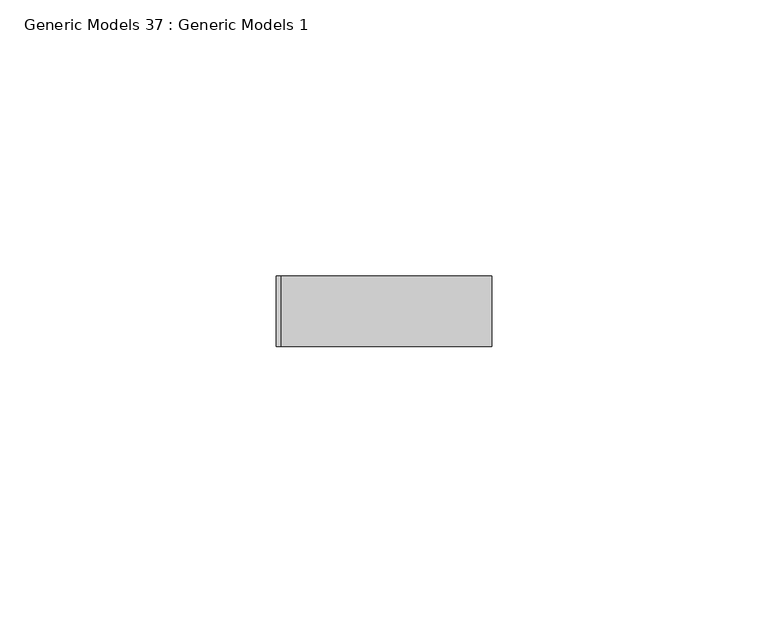
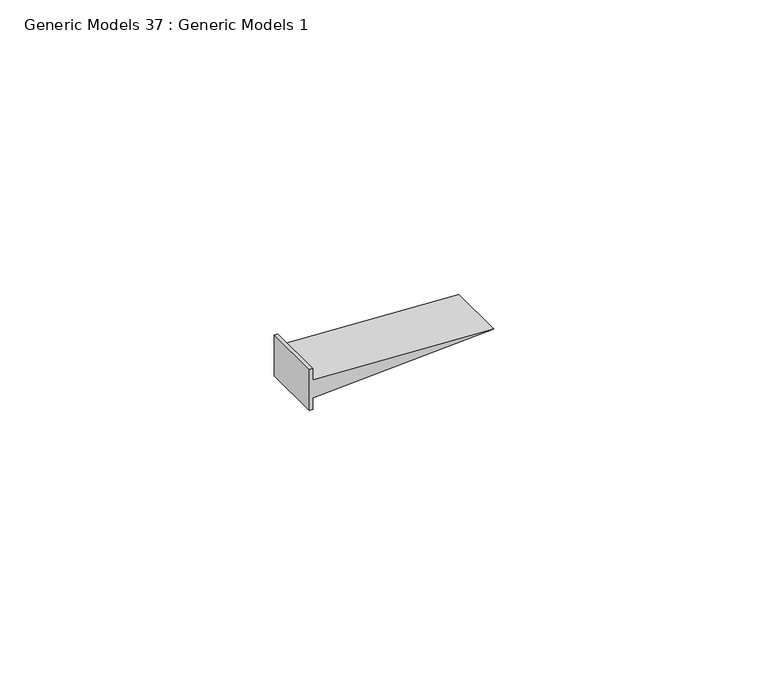
"""IFC4 building model written with IfcOpenShell, lengths in millimetres: proxy geometry, Generic Models 37 : Generic Models 1."""

from ifc_helpers import new_model, si_unit, frame, origin, place, context, project, spatial, polyline, outline, extrude, source, transform, mapped, element, save


def generic_models_37_generic_models_1_6ead30cd(model_context):
    return source(origin(), model_context, "Body", "SweptSolid", [
        extrude(outline(polyline([(2414.3721662, 49675.25625), (2405.2789662, 49675.25625), (2405.2789662, 49676.05), (2407.8288298, 49676.05), (2409.8255662, 49714.15), (2411.8223026, 49676.05), (2414.3721662, 49676.05), (2414.3721662, 49675.25625)])), frame((0.0, 565.15, 0.0), z_axis=(0.0, 1.0, 0.0), x_axis=(0.0, 0.0, 1.0)), (0.0, 0.0, 1.0), 12.7),
    ])


if __name__ == "__main__":
    model = new_model("IFC4")
    model_context = context("Model", 3, world=origin())
    ifc_project = project(units=[si_unit("LENGTHUNIT", "METRE", prefix="MILLI")], contexts=[model_context])
    site = spatial("IfcSite", under=ifc_project)
    building = spatial("IfcBuilding", under=site)
    placement = place(None, origin())
    generic_models_37_generic_models_1_shape = generic_models_37_generic_models_1_6ead30cd(model_context)
    element("IfcBuildingElementProxy", 1, Name="Generic Models 37 : Generic Models 1", ObjectType="Generic Models 37 : Generic Models 1", at=placement, inside=building, context=model_context, shape_type="MappedRepresentation", body=[
        mapped(generic_models_37_generic_models_1_shape, transform((0.0, 0.0, 0.0), x_axis=(1.0, 0.0, 0.0), y_axis=(0.0, 1.0, 0.0), z_axis=(0.0, 0.0, 1.0))),
    ])
    save(model, "model.ifc")

# Revit data of these elements
# Element 1 (IfcBuildingElementProxy, "Generic Models 37 : Generic Models 1")
#   Materials on its faces: "ATTACH GYPSUM BOARD TO STUDS AND NOT TO TOP TRACK"
# Materials
#   "ATTACH GYPSUM BOARD TO STUDS AND NOT TO TOP TRACK": class "Generic", colour RGB 48 48 48, transparency 0, Cost = 0
